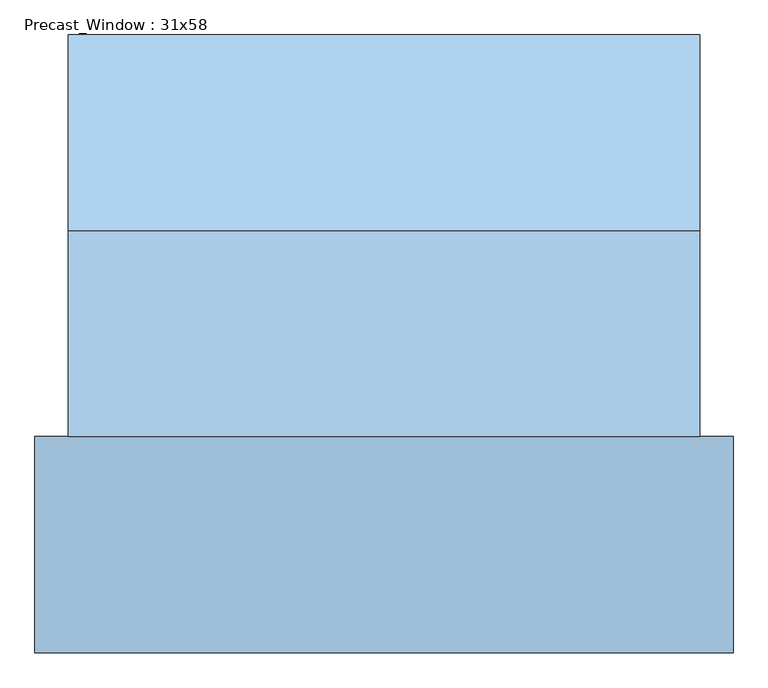
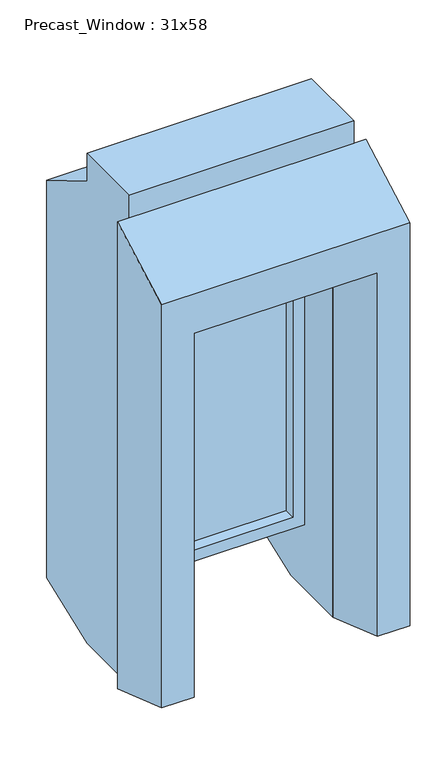
"""IFC4 building model written with IfcOpenShell, lengths in millimetres: window geometry, Precast_Window : 31x58."""

from ifc_helpers import new_model, si_unit, frame, origin, place, context, project, spatial, polyline, outline, extrude, faceted_brep, source, transform, mapped, element, save


def precast_window_31x58_d8990b54(model_context):
    return source(origin(), model_context, "Body", "SolidModel", [
        extrude(outline(polyline([(342.9, 106.3625), (-342.9, 106.3625), (-342.9, 125.4125), (342.9, 125.4125), (342.9, 106.3625)])), frame((0.0, 0.0, 1066.8), z_axis=(0.0, 0.0, 1.0), x_axis=(1.0, 0.0, 0.0)), (0.0, 0.0, 1.0), 1371.6),
        extrude(outline(polyline([(2489.2, -393.7), (1016.0, -393.7), (1016.0, 393.7), (2489.2, 393.7), (2489.2, -393.7)]), holes=[polyline([(2438.4, -342.9), (2438.4, 342.9), (1066.8, 342.9), (1066.8, -342.9), (2438.4, -342.9)])]), frame((0.0, 55.5625, 0.0), z_axis=(0.0, 1.0, 0.0), x_axis=(0.0, 0.0, 1.0)), (0.0, 0.0, 1.0), 101.6),
        faceted_brep([(482.6, 457.2, 838.2), (482.6, 457.2, 2641.6), (482.6, 157.1625, 2819.4), (482.6, 157.1625, 2946.4), (482.6, -157.1625, 2946.4), (482.6, -157.1625, 723.9), (482.6, 157.1625, 723.9), (393.7, -157.1625, 723.9), (-482.6, -157.1625, 2946.4), (-482.6, -157.1625, 723.9), (-393.7, -157.1625, 723.9), (-393.7, -157.1625, 2489.2), (393.7, -157.1625, 2489.2), (393.7, 457.2, 2489.2), (-393.7, 457.2, 2489.2), (-393.7, 457.2, 838.2), (-482.6, 457.2, 838.2), (-482.6, 457.2, 2641.6), (393.7, 457.2, 838.2), (393.7, 157.1625, 723.9), (-482.6, 157.1625, 723.9), (-482.6, 157.1625, 2946.4), (-482.6, 157.1625, 2819.4), (-393.7, 157.1625, 723.9)], [[[0, 1, 2, 3, 4, 5, 6]], [[7, 5, 4, 8, 9, 10, 11, 12]], [[13, 14, 15, 16, 17, 1, 0, 18]], [[12, 13, 18, 19, 7]], [[16, 20, 9, 8, 21, 22, 17]], [[14, 11, 10, 23, 15]], [[12, 11, 14, 13]], [[3, 21, 8, 4]], [[2, 22, 21, 3]], [[1, 17, 22, 2]], [[6, 19, 18, 0]], [[5, 7, 19, 6]], [[10, 9, 20, 23]], [[23, 20, 16, 15]]]),
        faceted_brep([(533.4, -157.1625, 723.9), (533.4, -157.1625, 2844.8), (533.4, -487.3625, 2667.0), (533.4, -487.3625, 838.2), (393.7, -487.3625, 838.2), (393.7, -157.1625, 723.9), (-533.4, -487.3625, 2667.0), (-533.4, -487.3625, 838.2), (-393.7, -487.3625, 838.2), (-393.7, -487.3625, 2489.2), (393.7, -487.3625, 2489.2), (393.7, -157.1625, 2489.2), (-393.7, -157.1625, 2489.2), (-393.7, -157.1625, 723.9), (-533.4, -157.1625, 723.9), (-533.4, -157.1625, 2844.8)], [[[0, 1, 2, 3]], [[3, 4, 5, 0]], [[4, 3, 2, 6, 7, 8, 9, 10]], [[11, 12, 13, 14, 15, 1, 0, 5]], [[10, 11, 5, 4]], [[14, 7, 6, 15]], [[8, 7, 14, 13]], [[12, 9, 8, 13]], [[1, 15, 6, 2]], [[10, 9, 12, 11]]]),
    ])


if __name__ == "__main__":
    model = new_model("IFC4")
    model_context = context("Model", 3, world=origin())
    ifc_project = project(units=[si_unit("LENGTHUNIT", "METRE", prefix="MILLI")], contexts=[model_context])
    site = spatial("IfcSite", under=ifc_project)
    building = spatial("IfcBuilding", under=site)
    placement = place(None, origin())
    precast_window_31x58_shape = precast_window_31x58_d8990b54(model_context)
    element("IfcWindow", 1, ObjectType="Precast_Window : 31x58", at=placement, inside=building, context=model_context, shape_type="MappedRepresentation", body=[
        mapped(precast_window_31x58_shape, transform((0.0, 0.0, 0.0), x_axis=(1.0, 0.0, 0.0), y_axis=(0.0, 1.0, 0.0), z_axis=(0.0, 0.0, 1.0))),
    ])
    save(model, "model.ifc")

# Revit data of these elements
# Type "Precast_Window : 31x58"
#   Type Mark = "24"
#   Analytic Construction = "<None>"
#   Height = 4' - 10"
#   Frame Width = 0' - 2"
#   Default Sill Height = 4' - 0"
#   Width = 2' - 7"
#   Precast Material = Stucco - Plaster Cement - Taupe
#   Frame Material = Metal Trim
#   Wall Closure = (empty or 0)
# Element 1 (IfcWindow, "Precast_Window : 31x58")
#   Materials on its faces: "Stucco - Plaster Cement - Taupe", "Metal Trim", "Glass"
# Materials
#   "Stucco - Plaster Cement - Taupe": class "Generic", colour RGB 137 123 107, transparency 0, Description = "Gypsum Wall Board", Cost = 0
#   "Metal Trim": class "Wood", colour RGB 151 137 121, transparency 0, Cost = 0
#   "Glass": class "Glass", colour RGB 218 227 224, transparency 0.85, Description = "Soda Lime Glass", Cost = 0
